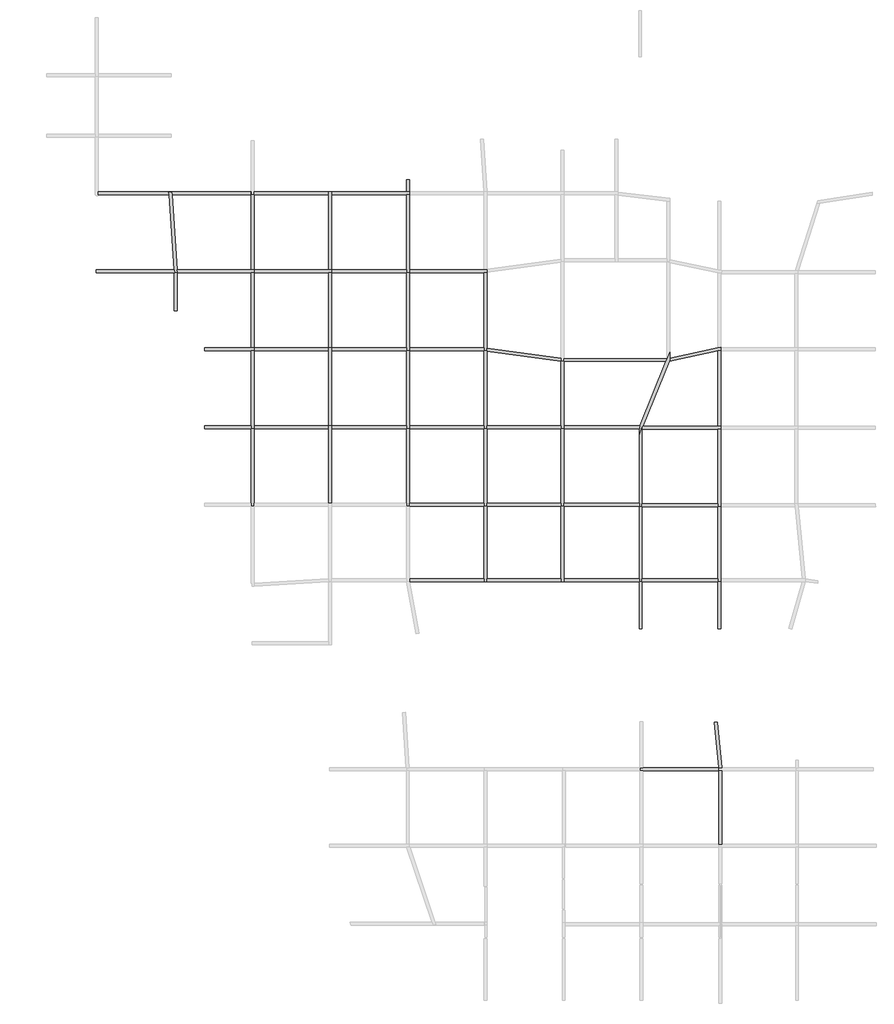
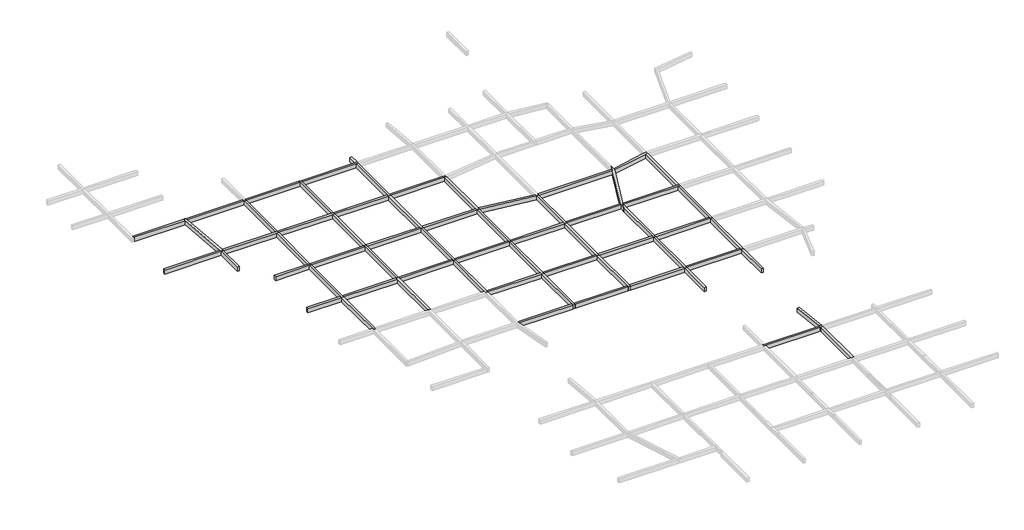
# One storey, part 2 of 8: 64 beams.
"""IFC4 building model written with IfcOpenShell, lengths in millimetres."""

from ifc_helpers import new_model, si_unit, frame, origin, place, context, project, spatial, polyline, outline, extrude, faceted_brep, element, save

model = new_model("IFC4")

# Units and contexts
model_context = context("Model", 3, world=origin())
ifc_project = project(units=[si_unit("LENGTHUNIT", "METRE", prefix="MILLI")], contexts=[model_context])

# Site, building, storey
site = spatial("IfcSite", under=ifc_project)
building = spatial("IfcBuilding", under=site)
storey = spatial("IfcBuildingStorey", under=building, Name="层高", Elevation=3300.0)

# Beams
placement = place(None, origin())
element("IfcBeam", 1, ObjectType="混凝土 - 矩形梁 : KL_beam", at=placement, inside=storey, context=model_context, shape_type="Brep", body=[
    faceted_brep([(70180.9452484, 119135.802002, 3300.0), (70480.2144635, 119156.7289441, 3300.0), (70460.6997743, 119435.802002, 3300.0), (69929.2560035, 127035.802002, 3300.0), (69908.2779599, 127335.802002, 3300.0), (69609.0087449, 127314.8750599, 3300.0), (69628.5234341, 127035.802002, 3300.0), (70159.9672049, 119435.802002, 3300.0), (70180.9452484, 119135.802002, 2700.0), (69609.0087449, 127314.8750599, 2700.0), (69628.5234341, 127035.802002, 2700.0), (70159.9672049, 119435.802002, 2700.0), (70480.2144635, 119156.7289441, 2700.0), (69908.2779599, 127335.802002, 2700.0), (69929.2560035, 127035.802002, 2700.0), (70460.6997743, 119435.802002, 2700.0)], [[[0, 1, 2, 3, 4, 5, 6, 7]], [[8, 0, 7, 6, 5, 9, 10, 11]], [[12, 8, 11, 10, 9, 13, 14, 15]], [[1, 12, 15, 14, 13, 4, 3, 2]], [[4, 13, 9, 5]], [[1, 0, 8, 12]]]),
])
element("IfcBeam", 2, ObjectType="混凝土 - 矩形梁 : KL_beam", at=placement, inside=storey, context=model_context, shape_type="Brep", body=[
    faceted_brep([(62233.8430954, 119135.802002, 3300.0), (70170.8225114, 119135.802002, 3300.0), (70180.9452484, 119135.802002, 3300.0), (70159.9672049, 119435.802002, 3300.0), (62233.8430954, 119435.802002, 3300.0), (62233.8430954, 119435.802002, 2700.0), (70159.9672049, 119435.802002, 2700.0), (70180.9452484, 119135.802002, 2700.0), (70170.8225114, 119135.802002, 2700.0), (62233.8430954, 119135.802002, 2700.0)], [[[0, 1, 2, 3, 4]], [[5, 4, 3, 6]], [[7, 8, 9, 5, 6]], [[2, 1, 0, 9, 8, 7]], [[0, 4, 5, 9]], [[3, 2, 7, 6]]]),
])
element("IfcBeam", 3, ObjectType="混凝土 - 矩形梁 : KL_beam", at=placement, inside=storey, context=model_context, shape_type="Brep", body=[
    faceted_brep([(70460.6997743, 119435.802002, 3300.0), (70480.2144635, 119156.7289441, 3300.0), (70180.9452484, 119135.802002, 3300.0), (70470.8225114, 119135.802002, 3300.0), (77970.8225114, 119135.802002, 3300.0), (78270.8225114, 119135.802002, 3300.0), (78270.8225114, 119435.802002, 3300.0), (77970.8225114, 119435.802002, 3300.0), (78270.8225114, 119135.802002, 2700.0), (70180.9452484, 119135.802002, 2700.0), (70470.8225114, 119135.802002, 2700.0), (77970.8225114, 119135.802002, 2700.0), (70480.2144635, 119156.7289441, 2700.0), (70460.6997743, 119435.802002, 2700.0), (77970.8225114, 119435.802002, 2700.0), (78270.8225114, 119435.802002, 2700.0)], [[[0, 1, 2, 3, 4, 5, 6, 7]], [[8, 5, 4, 3, 2, 9, 10, 11]], [[12, 13, 14, 15, 8, 11, 10, 9]], [[13, 0, 7, 6, 15, 14]], [[12, 1, 0, 13]], [[1, 12, 9, 2]], [[6, 5, 8, 15]]]),
])
element("IfcBeam", 4, ObjectType="混凝土 - 矩形梁 : KL_beam", at=placement, inside=storey, context=model_context, shape_type="Brep", body=[
    faceted_brep([(77970.8225114, 119435.802002, 3300.0), (78270.8225114, 119435.802002, 3300.0), (78270.8225114, 127035.802002, 3300.0), (77992.6046485, 127035.802002, 3300.0), (77992.6046485, 127335.802002, 3300.0), (77970.8225114, 127335.802002, 3300.0), (77970.8225114, 127035.802002, 3300.0), (78270.8225114, 119435.802002, 2700.0), (78270.8225114, 127035.802002, 2700.0), (77970.8225114, 119435.802002, 2700.0), (77970.8225114, 127035.802002, 2700.0), (77970.8225114, 127335.802002, 2700.0), (77992.6046485, 127335.802002, 2700.0), (77992.6046485, 127035.802002, 2700.0)], [[[0, 1, 2, 3, 4, 5, 6]], [[1, 7, 8, 2]], [[7, 9, 10, 11, 12, 13, 8]], [[5, 11, 10, 9, 0, 6]], [[3, 13, 12, 4]], [[1, 0, 9, 7]], [[11, 5, 4, 12]], [[13, 3, 2, 8]]]),
])
element("IfcBeam", 5, ObjectType="混凝土 - 矩形梁 : KL_beam", at=placement, inside=storey, context=model_context, shape_type="Brep", body=[
    faceted_brep([(86170.8225114, 119135.802002, 3300.0), (86170.8225114, 119435.802002, 3300.0), (85870.8225114, 119435.802002, 3300.0), (78270.8225114, 119435.802002, 3300.0), (78270.8225114, 119135.802002, 3300.0), (85870.8225114, 119135.802002, 3300.0), (86170.8225114, 119135.802002, 2700.0), (78270.8225114, 119135.802002, 2700.0), (85870.8225114, 119135.802002, 2700.0), (86170.8225114, 119435.802002, 2700.0), (78270.8225114, 119435.802002, 2700.0), (85870.8225114, 119435.802002, 2700.0)], [[[0, 1, 2, 3, 4, 5]], [[6, 0, 5, 4, 7, 8]], [[9, 6, 8, 7, 10, 11]], [[1, 9, 11, 10, 3, 2]], [[4, 3, 10, 7]], [[1, 0, 6, 9]]]),
])
element("IfcBeam", 6, ObjectType="混凝土 - 矩形梁 : KL_beam", at=placement, inside=storey, context=model_context, shape_type="Brep", body=[
    faceted_brep([(86170.8225114, 127335.802002, 3300.0), (85870.8225114, 127335.802002, 3300.0), (85870.8225114, 127035.802002, 3300.0), (85870.8225114, 119435.802002, 3300.0), (86170.8225114, 119435.802002, 3300.0), (86170.8225114, 127035.802002, 3300.0), (86170.8225114, 127335.802002, 2700.0), (86170.8225114, 119435.802002, 2700.0), (86170.8225114, 127035.802002, 2700.0), (85870.8225114, 127335.802002, 2700.0), (85870.8225114, 119435.802002, 2700.0), (85870.8225114, 127035.802002, 2700.0)], [[[0, 1, 2, 3, 4, 5]], [[6, 0, 5, 4, 7, 8]], [[9, 6, 8, 7, 10, 11]], [[1, 9, 11, 10, 3, 2]], [[4, 3, 10, 7]], [[1, 0, 6, 9]]]),
])
element("IfcBeam", 7, ObjectType="混凝土 - 矩形梁 : KL_beam", at=placement, inside=storey, context=model_context, shape_type="Brep", body=[
    faceted_brep([(94070.8225114, 127035.802002, 3300.0), (94070.8225114, 127335.802002, 3300.0), (93770.8225114, 127335.802002, 3300.0), (86170.8225114, 127335.802002, 3300.0), (86170.8225114, 127035.802002, 3300.0), (93770.8225114, 127035.802002, 3300.0), (94070.8225114, 127035.802002, 2700.0), (86170.8225114, 127035.802002, 2700.0), (93770.8225114, 127035.802002, 2700.0), (94070.8225114, 127335.802002, 2700.0), (86170.8225114, 127335.802002, 2700.0), (93770.8225114, 127335.802002, 2700.0)], [[[0, 1, 2, 3, 4, 5]], [[6, 0, 5, 4, 7, 8]], [[9, 6, 8, 7, 10, 11]], [[1, 9, 11, 10, 3, 2]], [[4, 3, 10, 7]], [[1, 0, 6, 9]]]),
])
element("IfcBeam", 8, ObjectType="混凝土 - 矩形梁 : KL_beam", at=placement, inside=storey, context=model_context, shape_type="Brep", body=[
    faceted_brep([(93770.8225114, 119135.802002, 3300.0), (94070.8225114, 119135.802002, 3300.0), (94070.8225114, 119435.802002, 3300.0), (94070.8225114, 127035.802002, 3300.0), (93770.8225114, 127035.802002, 3300.0), (93770.8225114, 119435.802002, 3300.0), (93770.8225114, 119135.802002, 2700.0), (93770.8225114, 127035.802002, 2700.0), (93770.8225114, 119435.802002, 2700.0), (94070.8225114, 119135.802002, 2700.0), (94070.8225114, 127035.802002, 2700.0), (94070.8225114, 119435.802002, 2700.0)], [[[0, 1, 2, 3, 4, 5]], [[6, 0, 5, 4, 7, 8]], [[9, 6, 8, 7, 10, 11]], [[1, 9, 11, 10, 3, 2]], [[4, 3, 10, 7]], [[1, 0, 6, 9]]]),
])
element("IfcBeam", 9, ObjectType="混凝土 - 矩形梁 : KL_beam", at=placement, inside=storey, context=model_context, shape_type="SweptSolid", body=[
    extrude(outline(polyline([(86170.8225114, 119135.802002), (86170.8225114, 119435.802002), (93770.8225114, 119435.802002), (93770.8225114, 119135.802002), (86170.8225114, 119135.802002)])), frame((0.0, 0.0, 2700.0), z_axis=(0.0, 0.0, 1.0), x_axis=(1.0, 0.0, 0.0)), (0.0, 0.0, 1.0), 600.0),
])
element("IfcBeam", 10, ObjectType="混凝土 - 矩形梁 : KL_beam", at=placement, inside=storey, context=model_context, shape_type="Brep", body=[
    faceted_brep([(101970.8225114, 119135.802002, 3300.0), (101970.8225114, 119155.4715744, 3300.0), (101970.8225114, 119435.802002, 3300.0), (101670.8225114, 119435.802002, 3300.0), (94070.8225114, 119435.802002, 3300.0), (94070.8225114, 119135.802002, 3300.0), (101670.8225114, 119135.802002, 3300.0), (101970.8225114, 119135.802002, 2700.0), (94070.8225114, 119135.802002, 2700.0), (101670.8225114, 119135.802002, 2700.0), (101970.8225114, 119435.802002, 2700.0), (101970.8225114, 119155.4715744, 2700.0), (94070.8225114, 119435.802002, 2700.0), (101670.8225114, 119435.802002, 2700.0)], [[[0, 1, 2, 3, 4, 5, 6]], [[7, 0, 6, 5, 8, 9]], [[10, 11, 7, 9, 8, 12, 13]], [[2, 10, 13, 12, 4, 3]], [[5, 4, 12, 8]], [[2, 1, 0, 7, 11, 10]]]),
])
element("IfcBeam", 11, ObjectType="混凝土 - 矩形梁 : KL_beam", at=placement, inside=storey, context=model_context, shape_type="SweptSolid", body=[
    extrude(outline(polyline([(93770.8225114, 128593.2738083), (94070.8225114, 128593.2738083), (94070.8225114, 127335.802002), (93770.8225114, 127335.802002), (93770.8225114, 128593.2738083)])), frame((0.0, 0.0, 2700.0), z_axis=(0.0, 0.0, 1.0), x_axis=(1.0, 0.0, 0.0)), (0.0, 0.0, 1.0), 600.0),
])
element("IfcBeam", 12, ObjectType="混凝土 - 矩形梁 : KL_beam", at=placement, inside=storey, context=model_context, shape_type="Brep", body=[
    faceted_brep([(70170.8225114, 115247.0451941, 3300.0), (70470.8225114, 115247.0451941, 3300.0), (70470.8225114, 119135.802002, 3300.0), (70180.9452484, 119135.802002, 3300.0), (70170.8225114, 119135.802002, 3300.0), (70170.8225114, 115247.0451941, 2700.0), (70170.8225114, 119135.802002, 2700.0), (70470.8225114, 115247.0451941, 2700.0), (70180.9452484, 119135.802002, 2700.0), (70470.8225114, 119135.802002, 2700.0)], [[[0, 1, 2, 3, 4]], [[5, 0, 4, 6]], [[7, 5, 6, 8, 9]], [[1, 7, 9, 2]], [[1, 0, 5, 7]], [[2, 9, 8, 6, 4, 3]]]),
])
element("IfcBeam", 13, ObjectType="混凝土 - 矩形梁 : KL_beam", at=placement, inside=storey, context=model_context, shape_type="Brep", body=[
    faceted_brep([(78270.8225114, 111177.0451941, 3300.0), (78270.8225114, 111477.0451941, 3300.0), (77970.8225114, 111477.0451941, 3300.0), (73233.8430954, 111477.0451941, 3300.0), (73233.8430954, 111177.0451941, 3300.0), (77970.8225114, 111177.0451941, 3300.0), (78270.8225114, 111177.0451941, 2700.0), (73233.8430954, 111177.0451941, 2700.0), (77970.8225114, 111177.0451941, 2700.0), (78270.8225114, 111477.0451941, 2700.0), (73233.8430954, 111477.0451941, 2700.0), (77970.8225114, 111477.0451941, 2700.0)], [[[0, 1, 2, 3, 4, 5]], [[6, 0, 5, 4, 7, 8]], [[9, 6, 8, 7, 10, 11]], [[1, 9, 11, 10, 3, 2]], [[4, 3, 10, 7]], [[1, 0, 6, 9]]]),
])
element("IfcBeam", 14, ObjectType="混凝土 - 矩形梁 : KL_beam", at=placement, inside=storey, context=model_context, shape_type="SweptSolid", body=[
    extrude(outline(polyline([(77970.8225114, 119135.802002), (78270.8225114, 119135.802002), (78270.8225114, 111477.0451941), (77970.8225114, 111477.0451941), (77970.8225114, 119135.802002)])), frame((0.0, 0.0, 2700.0), z_axis=(0.0, 0.0, 1.0), x_axis=(1.0, 0.0, 0.0)), (0.0, 0.0, 1.0), 600.0),
])
element("IfcBeam", 15, ObjectType="混凝土 - 矩形梁 : KL_beam", at=placement, inside=storey, context=model_context, shape_type="Brep", body=[
    faceted_brep([(77970.8225114, 103277.0451941, 3300.0), (78270.8225114, 103277.0451941, 3300.0), (78270.8225114, 103577.0451941, 3300.0), (78270.8225114, 111177.0451941, 3300.0), (77970.8225114, 111177.0451941, 3300.0), (77970.8225114, 103577.0451941, 3300.0), (77970.8225114, 103277.0451941, 2700.0), (77970.8225114, 111177.0451941, 2700.0), (77970.8225114, 103577.0451941, 2700.0), (78270.8225114, 103277.0451941, 2700.0), (78270.8225114, 111177.0451941, 2700.0), (78270.8225114, 103577.0451941, 2700.0)], [[[0, 1, 2, 3, 4, 5]], [[6, 0, 5, 4, 7, 8]], [[9, 6, 8, 7, 10, 11]], [[1, 9, 11, 10, 3, 2]], [[4, 3, 10, 7]], [[1, 0, 6, 9]]]),
])
element("IfcBeam", 16, ObjectType="混凝土 - 矩形梁 : KL_beam", at=placement, inside=storey, context=model_context, shape_type="SweptSolid", body=[
    extrude(outline(polyline([(73233.8430954, 103277.0451941), (73233.8430954, 103577.0451941), (77970.8225114, 103577.0451941), (77970.8225114, 103277.0451941), (73233.8430954, 103277.0451941)])), frame((0.0, 0.0, 2700.0), z_axis=(0.0, 0.0, 1.0), x_axis=(1.0, 0.0, 0.0)), (0.0, 0.0, 1.0), 600.0),
])
element("IfcBeam", 17, ObjectType="混凝土 - 矩形梁 : KL_beam", at=placement, inside=storey, context=model_context, shape_type="Brep", body=[
    faceted_brep([(77970.8225114, 95377.0451941, 3300.0), (78270.8225114, 95377.0451941, 3300.0), (78270.8225114, 95677.0451941, 3300.0), (78270.8225114, 103277.0451941, 3300.0), (77970.8225114, 103277.0451941, 3300.0), (77970.8225114, 95677.0451941, 3300.0), (77970.8225114, 95377.0451941, 2700.0), (77970.8225114, 103277.0451941, 2700.0), (77970.8225114, 95677.0451941, 2700.0), (78270.8225114, 95377.0451941, 2700.0), (78270.8225114, 103277.0451941, 2700.0), (78270.8225114, 95677.0451941, 2700.0)], [[[0, 1, 2, 3, 4, 5]], [[6, 0, 5, 4, 7, 8]], [[9, 6, 8, 7, 10, 11]], [[1, 9, 11, 10, 3, 2]], [[4, 3, 10, 7]], [[1, 0, 6, 9]]]),
])
element("IfcBeam", 18, ObjectType="混凝土 - 矩形梁 : KL_beam", at=placement, inside=storey, context=model_context, shape_type="Brep", body=[
    faceted_brep([(86170.8225114, 103577.0451941, 3300.0), (85870.8225114, 103577.0451941, 3300.0), (85870.8225114, 103277.0451941, 3300.0), (85870.8225114, 95677.0451941, 3300.0), (86170.8225114, 95677.0451941, 3300.0), (86170.8225114, 103277.0451941, 3300.0), (86170.8225114, 103577.0451941, 2700.0), (86170.8225114, 95677.0451941, 2700.0), (86170.8225114, 103277.0451941, 2700.0), (85870.8225114, 103577.0451941, 2700.0), (85870.8225114, 95677.0451941, 2700.0), (85870.8225114, 103277.0451941, 2700.0)], [[[0, 1, 2, 3, 4, 5]], [[6, 0, 5, 4, 7, 8]], [[9, 6, 8, 7, 10, 11]], [[1, 9, 11, 10, 3, 2]], [[1, 0, 6, 9]], [[4, 3, 10, 7]]]),
])
element("IfcBeam", 19, ObjectType="混凝土 - 矩形梁 : KL_beam", at=placement, inside=storey, context=model_context, shape_type="Brep", body=[
    faceted_brep([(86170.8225114, 111477.0451941, 3300.0), (85870.8225114, 111477.0451941, 3300.0), (85870.8225114, 111177.0451941, 3300.0), (85870.8225114, 103577.0451941, 3300.0), (86170.8225114, 103577.0451941, 3300.0), (86170.8225114, 111177.0451941, 3300.0), (86170.8225114, 111477.0451941, 2700.0), (86170.8225114, 103577.0451941, 2700.0), (86170.8225114, 111177.0451941, 2700.0), (85870.8225114, 111477.0451941, 2700.0), (85870.8225114, 103577.0451941, 2700.0), (85870.8225114, 111177.0451941, 2700.0)], [[[0, 1, 2, 3, 4, 5]], [[6, 0, 5, 4, 7, 8]], [[9, 6, 8, 7, 10, 11]], [[1, 9, 11, 10, 3, 2]], [[1, 0, 6, 9]], [[4, 3, 10, 7]]]),
])
element("IfcBeam", 20, ObjectType="混凝土 - 矩形梁 : KL_beam", at=placement, inside=storey, context=model_context, shape_type="SweptSolid", body=[
    extrude(outline(polyline([(85870.8225114, 119135.802002), (86170.8225114, 119135.802002), (86170.8225114, 111477.0451941), (85870.8225114, 111477.0451941), (85870.8225114, 119135.802002)])), frame((0.0, 0.0, 2700.0), z_axis=(0.0, 0.0, 1.0), x_axis=(1.0, 0.0, 0.0)), (0.0, 0.0, 1.0), 600.0),
])
element("IfcBeam", 21, ObjectType="混凝土 - 矩形梁 : KL_beam", at=placement, inside=storey, context=model_context, shape_type="Brep", body=[
    faceted_brep([(93770.8225114, 111177.0451941, 3300.0), (94070.8225114, 111177.0451941, 3300.0), (94070.8225114, 111477.0451941, 3300.0), (94070.8225114, 119135.802002, 3300.0), (93770.8225114, 119135.802002, 3300.0), (93770.8225114, 111477.0451941, 3300.0), (93770.8225114, 111177.0451941, 2700.0), (93770.8225114, 119135.802002, 2700.0), (93770.8225114, 111477.0451941, 2700.0), (94070.8225114, 111177.0451941, 2700.0), (94070.8225114, 119135.802002, 2700.0), (94070.8225114, 111477.0451941, 2700.0)], [[[0, 1, 2, 3, 4, 5]], [[6, 0, 5, 4, 7, 8]], [[9, 6, 8, 7, 10, 11]], [[1, 9, 11, 10, 3, 2]], [[4, 3, 10, 7]], [[1, 0, 6, 9]]]),
])
element("IfcBeam", 22, ObjectType="混凝土 - 矩形梁 : KL_beam", at=placement, inside=storey, context=model_context, shape_type="Brep", body=[
    faceted_brep([(93770.8225114, 103277.0451941, 3300.0), (94070.8225114, 103277.0451941, 3300.0), (94070.8225114, 103577.0451941, 3300.0), (94070.8225114, 111177.0451941, 3300.0), (93770.8225114, 111177.0451941, 3300.0), (93770.8225114, 103577.0451941, 3300.0), (93770.8225114, 103277.0451941, 2700.0), (93770.8225114, 111177.0451941, 2700.0), (93770.8225114, 103577.0451941, 2700.0), (94070.8225114, 103277.0451941, 2700.0), (94070.8225114, 111177.0451941, 2700.0), (94070.8225114, 103577.0451941, 2700.0)], [[[0, 1, 2, 3, 4, 5]], [[6, 0, 5, 4, 7, 8]], [[9, 6, 8, 7, 10, 11]], [[1, 9, 11, 10, 3, 2]], [[4, 3, 10, 7]], [[1, 0, 6, 9]]]),
])
element("IfcBeam", 23, ObjectType="混凝土 - 矩形梁 : KL_beam", at=placement, inside=storey, context=model_context, shape_type="Brep", body=[
    faceted_brep([(93770.8225114, 95377.0451941, 3300.0), (94070.8225114, 95377.0451941, 3300.0), (94070.8225114, 95677.0451941, 3300.0), (94070.8225114, 103277.0451941, 3300.0), (93770.8225114, 103277.0451941, 3300.0), (93770.8225114, 95677.0451941, 3300.0), (93770.8225114, 95377.0451941, 2700.0), (93770.8225114, 103277.0451941, 2700.0), (93770.8225114, 95677.0451941, 2700.0), (94070.8225114, 95377.0451941, 2700.0), (94070.8225114, 103277.0451941, 2700.0), (94070.8225114, 95677.0451941, 2700.0)], [[[0, 1, 2, 3, 4, 5]], [[6, 0, 5, 4, 7, 8]], [[9, 6, 8, 7, 10, 11]], [[1, 9, 11, 10, 3, 2]], [[4, 3, 10, 7]], [[1, 0, 6, 9]]]),
])
element("IfcBeam", 24, ObjectType="混凝土 - 矩形梁 : KL_beam", at=placement, inside=storey, context=model_context, shape_type="Brep", body=[
    faceted_brep([(101670.8225114, 111177.0451941, 3300.0), (101970.8225114, 111177.0451941, 3300.0), (101970.8225114, 111457.869772, 3300.0), (101970.8225114, 119135.802002, 3300.0), (101670.8225114, 119135.802002, 3300.0), (101670.8225114, 111477.0451941, 3300.0), (101670.8225114, 111177.0451941, 2700.0), (101670.8225114, 119135.802002, 2700.0), (101670.8225114, 111477.0451941, 2700.0), (101970.8225114, 111177.0451941, 2700.0), (101970.8225114, 119135.802002, 2700.0), (101970.8225114, 111457.869772, 2700.0)], [[[0, 1, 2, 3, 4, 5]], [[6, 0, 5, 4, 7, 8]], [[9, 6, 8, 7, 10, 11]], [[1, 9, 11, 10, 3, 2]], [[4, 3, 10, 7]], [[1, 0, 6, 9]]]),
])
element("IfcBeam", 25, ObjectType="混凝土 - 矩形梁 : KL_beam", at=placement, inside=storey, context=model_context, shape_type="Brep", body=[
    faceted_brep([(101670.8225114, 103277.0451941, 3300.0), (101970.8225114, 103277.0451941, 3300.0), (101970.8225114, 103577.0451941, 3300.0), (101970.8225114, 111155.0591624, 3300.0), (101970.8225114, 111177.0451941, 3300.0), (101670.8225114, 111177.0451941, 3300.0), (101670.8225114, 103577.0451941, 3300.0), (101670.8225114, 103277.0451941, 2700.0), (101670.8225114, 111177.0451941, 2700.0), (101670.8225114, 103577.0451941, 2700.0), (101970.8225114, 103277.0451941, 2700.0), (101970.8225114, 111177.0451941, 2700.0), (101970.8225114, 111155.0591624, 2700.0), (101970.8225114, 103577.0451941, 2700.0)], [[[0, 1, 2, 3, 4, 5, 6]], [[7, 0, 6, 5, 8, 9]], [[10, 7, 9, 8, 11, 12, 13]], [[1, 10, 13, 12, 11, 4, 3, 2]], [[5, 4, 11, 8]], [[1, 0, 7, 10]]]),
])
element("IfcBeam", 26, ObjectType="混凝土 - 矩形梁 : KL_beam", at=placement, inside=storey, context=model_context, shape_type="Brep", body=[
    faceted_brep([(101670.8225114, 95377.0451941, 3300.0), (101970.8225114, 95377.0451941, 3300.0), (101970.8225114, 95677.0451941, 3300.0), (101970.8225114, 103277.0451941, 3300.0), (101670.8225114, 103277.0451941, 3300.0), (101670.8225114, 95677.0451941, 3300.0), (101670.8225114, 95377.0451941, 2700.0), (101670.8225114, 103277.0451941, 2700.0), (101670.8225114, 95677.0451941, 2700.0), (101970.8225114, 95377.0451941, 2700.0), (101970.8225114, 103277.0451941, 2700.0), (101970.8225114, 95677.0451941, 2700.0)], [[[0, 1, 2, 3, 4, 5]], [[6, 0, 5, 4, 7, 8]], [[9, 6, 8, 7, 10, 11]], [[1, 9, 11, 10, 3, 2]], [[4, 3, 10, 7]], [[1, 0, 6, 9]]]),
])
element("IfcBeam", 27, ObjectType="混凝土 - 矩形梁 : KL_beam", at=placement, inside=storey, context=model_context, shape_type="Brep", body=[
    faceted_brep([(101670.8225114, 87731.7102801, 3300.0), (101970.8225114, 87731.7102801, 3300.0), (101970.8225114, 88031.7102801, 3300.0), (101970.8225114, 95377.0451941, 3300.0), (101670.8225114, 95377.0451941, 3300.0), (101670.8225114, 88031.7102801, 3300.0), (101670.8225114, 87731.7102801, 2700.0), (101670.8225114, 95377.0451941, 2700.0), (101670.8225114, 88031.7102801, 2700.0), (101970.8225114, 87731.7102801, 2700.0), (101970.8225114, 95377.0451941, 2700.0), (101970.8225114, 88031.7102801, 2700.0)], [[[0, 1, 2, 3, 4, 5]], [[6, 0, 5, 4, 7, 8]], [[9, 6, 8, 7, 10, 11]], [[1, 9, 11, 10, 3, 2]], [[4, 3, 10, 7]], [[1, 0, 6, 9]]]),
])
element("IfcBeam", 28, ObjectType="混凝土 - 矩形梁 : KL_beam", at=placement, inside=storey, context=model_context, shape_type="Brep", body=[
    faceted_brep([(109470.8225114, 103277.0451941, 3300.0), (109770.8225114, 103277.0451941, 3300.0), (109770.8225114, 103577.0451941, 3300.0), (109770.8225114, 110106.8473936, 3300.0), (109470.8225114, 110106.8473936, 3300.0), (109470.8225114, 103577.0451941, 3300.0), (109470.8225114, 103277.0451941, 2700.0), (109470.8225114, 110106.8473936, 2700.0), (109470.8225114, 103577.0451941, 2700.0), (109770.8225114, 103277.0451941, 2700.0), (109770.8225114, 110106.8473936, 2700.0), (109770.8225114, 103577.0451941, 2700.0)], [[[0, 1, 2, 3, 4, 5]], [[6, 0, 5, 4, 7, 8]], [[9, 6, 8, 7, 10, 11]], [[1, 9, 11, 10, 3, 2]], [[4, 3, 10, 7]], [[1, 0, 6, 9]]]),
])
element("IfcBeam", 29, ObjectType="混凝土 - 矩形梁 : KL_beam", at=placement, inside=storey, context=model_context, shape_type="Brep", body=[
    faceted_brep([(109470.8225114, 95377.0451941, 3300.0), (109770.8225114, 95377.0451941, 3300.0), (109770.8225114, 95677.0451941, 3300.0), (109770.8225114, 103277.0451941, 3300.0), (109470.8225114, 103277.0451941, 3300.0), (109470.8225114, 95677.0451941, 3300.0), (109470.8225114, 95377.0451941, 2700.0), (109470.8225114, 103277.0451941, 2700.0), (109470.8225114, 95677.0451941, 2700.0), (109770.8225114, 95377.0451941, 2700.0), (109770.8225114, 103277.0451941, 2700.0), (109770.8225114, 95677.0451941, 2700.0)], [[[0, 1, 2, 3, 4, 5]], [[6, 0, 5, 4, 7, 8]], [[9, 6, 8, 7, 10, 11]], [[1, 9, 11, 10, 3, 2]], [[4, 3, 10, 7]], [[1, 0, 6, 9]]]),
])
element("IfcBeam", 30, ObjectType="混凝土 - 矩形梁 : KL_beam", at=placement, inside=storey, context=model_context, shape_type="Brep", body=[
    faceted_brep([(109470.8225114, 87731.7102801, 3300.0), (109770.8225114, 87731.7102801, 3300.0), (109770.8225114, 88031.7102801, 3300.0), (109770.8225114, 95377.0451941, 3300.0), (109470.8225114, 95377.0451941, 3300.0), (109470.8225114, 88031.7102801, 3300.0), (109470.8225114, 87731.7102801, 2700.0), (109470.8225114, 95377.0451941, 2700.0), (109470.8225114, 88031.7102801, 2700.0), (109770.8225114, 87731.7102801, 2700.0), (109770.8225114, 95377.0451941, 2700.0), (109770.8225114, 88031.7102801, 2700.0)], [[[0, 1, 2, 3, 4, 5]], [[6, 0, 5, 4, 7, 8]], [[9, 6, 8, 7, 10, 11]], [[1, 9, 11, 10, 3, 2]], [[4, 3, 10, 7]], [[1, 0, 6, 9]]]),
])
element("IfcBeam", 31, ObjectType="混凝土 - 矩形梁 : KL_beam", at=placement, inside=storey, context=model_context, shape_type="Brep", body=[
    faceted_brep([(117426.2900999, 103411.1618028, 3300.0), (117426.2900999, 103277.0451941, 3300.0), (117426.2900999, 102617.7429892, 3300.0), (117726.2900999, 103352.2587574, 3300.0), (117799.5839067, 103531.7102801, 3300.0), (120493.1632599, 110126.6319733, 3300.0), (120534.3184952, 110227.3958709, 3300.0), (120534.3184952, 110442.081967, 3300.0), (120534.3184952, 111020.8146845, 3300.0), (120234.3184952, 110286.2989162, 3300.0), (120161.0246884, 110106.8473936, 3300.0), (117494.0422429, 103577.0451941, 3300.0), (117426.2900999, 103411.1618028, 2700.0), (120534.3184952, 111020.8146845, 2700.0), (120234.3184952, 110286.2989162, 2700.0), (120161.0246884, 110106.8473936, 2700.0), (117494.0422429, 103577.0451941, 2700.0), (117426.2900999, 102617.7429892, 2700.0), (117426.2900999, 103277.0451941, 2700.0), (120534.3184952, 110442.081967, 2700.0), (120534.3184952, 110227.3958709, 2700.0), (120493.1632599, 110126.6319733, 2700.0), (117799.5839067, 103531.7102801, 2700.0), (117726.2900999, 103352.2587574, 2700.0)], [[[0, 1, 2, 3, 4, 5, 6, 7, 8, 9, 10, 11]], [[12, 0, 11, 10, 9, 8, 13, 14, 15, 16]], [[17, 18, 12, 16, 15, 14, 13, 19, 20, 21, 22, 23]], [[2, 17, 23, 22, 21, 20, 6, 5, 4, 3]], [[2, 1, 0, 12, 18, 17]], [[8, 7, 6, 20, 19, 13]]]),
])
element("IfcBeam", 32, ObjectType="混凝土 - 矩形梁 : KL_beam", at=placement, inside=storey, context=model_context, shape_type="Brep", body=[
    faceted_brep([(117426.2900999, 95331.7102801, 3300.0), (117726.2900999, 95331.7102801, 3300.0), (117726.2900999, 95631.7102801, 3300.0), (117726.2900999, 103231.7102801, 3300.0), (117726.2900999, 103352.2587574, 3300.0), (117426.2900999, 102617.7429892, 3300.0), (117426.2900999, 95677.0451941, 3300.0), (117426.2900999, 95377.0451941, 3300.0), (117426.2900999, 95331.7102801, 2700.0), (117426.2900999, 102617.7429892, 2700.0), (117426.2900999, 95677.0451941, 2700.0), (117426.2900999, 95377.0451941, 2700.0), (117726.2900999, 95331.7102801, 2700.0), (117726.2900999, 103352.2587574, 2700.0), (117726.2900999, 103231.7102801, 2700.0), (117726.2900999, 95631.7102801, 2700.0)], [[[0, 1, 2, 3, 4, 5, 6, 7]], [[8, 0, 7, 6, 5, 9, 10, 11]], [[12, 8, 11, 10, 9, 13, 14, 15]], [[1, 12, 15, 14, 13, 4, 3, 2]], [[5, 4, 13, 9]], [[1, 0, 8, 12]]]),
])
element("IfcBeam", 33, ObjectType="混凝土 - 矩形梁 : KL_beam", at=placement, inside=storey, context=model_context, shape_type="Brep", body=[
    faceted_brep([(117426.2900999, 87731.7102801, 3300.0), (117726.2900999, 87731.7102801, 3300.0), (117726.2900999, 88031.7102801, 3300.0), (117726.2900999, 95331.7102801, 3300.0), (117426.2900999, 95331.7102801, 3300.0), (117426.2900999, 88031.7102801, 3300.0), (117426.2900999, 87731.7102801, 2700.0), (117426.2900999, 95331.7102801, 2700.0), (117426.2900999, 88031.7102801, 2700.0), (117726.2900999, 87731.7102801, 2700.0), (117726.2900999, 95331.7102801, 2700.0), (117726.2900999, 88031.7102801, 2700.0)], [[[0, 1, 2, 3, 4, 5]], [[6, 0, 5, 4, 7, 8]], [[9, 6, 8, 7, 10, 11]], [[1, 9, 11, 10, 3, 2]], [[4, 3, 10, 7]], [[1, 0, 6, 9]]]),
])
element("IfcBeam", 34, ObjectType="混凝土 - 矩形梁 : KL_beam", at=placement, inside=storey, context=model_context, shape_type="SweptSolid", body=[
    extrude(outline(polyline([(117726.2900999, 82948.5269181), (117426.2900999, 82948.5269181), (117426.2900999, 87731.7102801), (117726.2900999, 87731.7102801), (117726.2900999, 82948.5269181)])), frame((0.0, 0.0, 2700.0), z_axis=(0.0, 0.0, 1.0), x_axis=(1.0, 0.0, 0.0)), (0.0, 0.0, 1.0), 600.0),
])
element("IfcBeam", 35, ObjectType="混凝土 - 矩形梁 : KL_beam", at=placement, inside=storey, context=model_context, shape_type="SweptSolid", body=[
    extrude(outline(polyline([(109770.8225114, 110106.8473936), (109770.8225114, 110406.8473936), (120234.3184952, 110406.8473936), (120234.3184952, 110286.2989162), (120161.0246884, 110106.8473936), (109770.8225114, 110106.8473936)])), frame((0.0, 0.0, 2700.0), z_axis=(0.0, 0.0, 1.0), x_axis=(1.0, 0.0, 0.0)), (0.0, 0.0, 1.0), 600.0),
])
element("IfcBeam", 36, ObjectType="混凝土 - 矩形梁 : KL_beam", at=placement, inside=storey, context=model_context, shape_type="Brep", body=[
    faceted_brep([(120534.3184952, 110227.3958709, 3300.0), (120493.1632599, 110126.6319733, 3300.0), (125448.8238726, 111179.9901539, 3300.0), (125748.8238726, 111243.7571224, 3300.0), (125748.8238726, 111515.2247274, 3300.0), (125748.8238726, 111550.4593009, 3300.0), (125448.8238726, 111486.6923324, 3300.0), (120534.3184952, 110442.081967, 3300.0), (120534.3184952, 110406.8473936, 3300.0), (120493.1632599, 110126.6319733, 2700.0), (125448.8238726, 111179.9901539, 2700.0), (125748.8238726, 111243.7571224, 2700.0), (120534.3184952, 110227.3958709, 2700.0), (120534.3184952, 110406.8473936, 2700.0), (120534.3184952, 110442.081967, 2700.0), (125448.8238726, 111486.6923324, 2700.0), (125748.8238726, 111550.4593009, 2700.0), (125748.8238726, 111515.2247274, 2700.0)], [[[0, 1, 2, 3, 4, 5, 6, 7, 8]], [[1, 9, 10, 11, 3, 2]], [[9, 12, 13, 14, 15, 16, 17, 11, 10]], [[14, 7, 6, 5, 16, 15]], [[0, 12, 9, 1]], [[12, 0, 8, 7, 14, 13]], [[5, 4, 3, 11, 17, 16]]]),
])
element("IfcBeam", 37, ObjectType="混凝土 - 矩形梁 : KL_beam", at=placement, inside=storey, context=model_context, shape_type="Brep", body=[
    faceted_brep([(125748.8238726, 103231.7102801, 3300.0), (125748.8238726, 103531.7102801, 3300.0), (125448.8238726, 103531.7102801, 3300.0), (117799.5839067, 103531.7102801, 3300.0), (117726.2900999, 103352.2587574, 3300.0), (117726.2900999, 103231.7102801, 3300.0), (125448.8238728, 103231.7102801, 3300.0), (125748.8238726, 103231.7102801, 2700.0), (117726.2900999, 103231.7102801, 2700.0), (125448.8238728, 103231.7102801, 2700.0), (125748.8238726, 103531.7102801, 2700.0), (117726.2900999, 103352.2587574, 2700.0), (117799.5839067, 103531.7102801, 2700.0), (125448.8238726, 103531.7102801, 2700.0)], [[[0, 1, 2, 3, 4, 5, 6]], [[7, 0, 6, 5, 8, 9]], [[10, 7, 9, 8, 11, 12, 13]], [[12, 3, 2, 1, 10, 13]], [[3, 12, 11, 4]], [[5, 4, 11, 8]], [[1, 0, 7, 10]]]),
])
element("IfcBeam", 38, ObjectType="混凝土 - 矩形梁 : KL_beam", at=placement, inside=storey, context=model_context, shape_type="Brep", body=[
    faceted_brep([(125748.8238726, 111243.7571224, 3300.0), (125448.8238726, 111179.9901539, 3300.0), (125448.8238726, 103531.7102801, 3300.0), (125748.8238726, 103531.7102801, 3300.0), (125748.8238726, 111215.2247274, 3300.0), (125448.8238726, 111179.9901539, 2700.0), (125448.8238726, 103531.7102801, 2700.0), (125748.8238726, 111243.7571224, 2700.0), (125748.8238726, 111215.2247274, 2700.0), (125748.8238726, 103531.7102801, 2700.0)], [[[0, 1, 2, 3, 4]], [[1, 5, 6, 2]], [[5, 7, 8, 9, 6]], [[7, 0, 4, 3, 9, 8]], [[1, 0, 7, 5]], [[3, 2, 6, 9]]]),
])
element("IfcBeam", 39, ObjectType="混凝土 - 矩形梁 : KL_beam", at=placement, inside=storey, context=model_context, shape_type="Brep", body=[
    faceted_brep([(125448.8238728, 95331.7102801, 3300.0), (125748.8238728, 95331.7102801, 3300.0), (125748.8238728, 95631.7102801, 3300.0), (125748.8238728, 103231.7102801, 3300.0), (125448.8238728, 103231.7102801, 3300.0), (125448.8238728, 95631.7102801, 3300.0), (125448.8238728, 95331.7102801, 2700.0), (125448.8238728, 103231.7102801, 2700.0), (125448.8238728, 95631.7102801, 2700.0), (125748.8238728, 95331.7102801, 2700.0), (125748.8238728, 103231.7102801, 2700.0), (125748.8238728, 95631.7102801, 2700.0)], [[[0, 1, 2, 3, 4, 5]], [[6, 0, 5, 4, 7, 8]], [[9, 6, 8, 7, 10, 11]], [[1, 9, 11, 10, 3, 2]], [[4, 3, 10, 7]], [[1, 0, 6, 9]]]),
])
element("IfcBeam", 40, ObjectType="混凝土 - 矩形梁 : KL_beam", at=placement, inside=storey, context=model_context, shape_type="SweptSolid", body=[
    extrude(outline(polyline([(117726.2900999, 95331.7102801), (117726.2900999, 95631.7102801), (125448.8238728, 95631.7102801), (125448.8238728, 95331.7102801), (117726.2900999, 95331.7102801)])), frame((0.0, 0.0, 2700.0), z_axis=(0.0, 0.0, 1.0), x_axis=(1.0, 0.0, 0.0)), (0.0, 0.0, 1.0), 600.0),
])
element("IfcBeam", 41, ObjectType="混凝土 - 矩形梁 : KL_beam", at=placement, inside=storey, context=model_context, shape_type="Brep", body=[
    faceted_brep([(125448.8238729, 87731.7102801, 3300.0), (125748.8238729, 87731.7102801, 3300.0), (125748.8238729, 88031.7102801, 3300.0), (125748.8238728, 95331.7102801, 3300.0), (125448.8238728, 95331.7102801, 3300.0), (125448.8238729, 88031.7102801, 3300.0), (125448.8238729, 87731.7102801, 2700.0), (125448.8238728, 95331.7102801, 2700.0), (125448.8238729, 88031.7102801, 2700.0), (125748.8238729, 87731.7102801, 2700.0), (125748.8238728, 95331.7102801, 2700.0), (125748.8238729, 88031.7102801, 2700.0)], [[[0, 1, 2, 3, 4, 5]], [[6, 0, 5, 4, 7, 8]], [[9, 6, 8, 7, 10, 11]], [[1, 9, 11, 10, 3, 2]], [[4, 3, 10, 7]], [[1, 0, 6, 9]]]),
])
element("IfcBeam", 42, ObjectType="混凝土 - 矩形梁 : KL_beam", at=placement, inside=storey, context=model_context, shape_type="SweptSolid", body=[
    extrude(outline(polyline([(117726.2900999, 87731.7102801), (117726.2900999, 88031.7102801), (125448.8238729, 88031.7102801), (125448.8238729, 87731.7102801), (117726.2900999, 87731.7102801)])), frame((0.0, 0.0, 2700.0), z_axis=(0.0, 0.0, 1.0), x_axis=(1.0, 0.0, 0.0)), (0.0, 0.0, 1.0), 600.0),
])
element("IfcBeam", 43, ObjectType="混凝土 - 矩形梁 : KL_beam", at=placement, inside=storey, context=model_context, shape_type="SweptSolid", body=[
    extrude(outline(polyline([(125748.8238729, 82948.5269181), (125448.8238729, 82948.5269181), (125448.8238729, 87731.7102801), (125748.8238729, 87731.7102801), (125748.8238729, 82948.5269181)])), frame((0.0, 0.0, 2700.0), z_axis=(0.0, 0.0, 1.0), x_axis=(1.0, 0.0, 0.0)), (0.0, 0.0, 1.0), 600.0),
])
element("IfcBeam", 44, ObjectType="混凝土 - 矩形梁 : KL_beam", at=placement, inside=storey, context=model_context, shape_type="Brep", body=[
    faceted_brep([(125476.4248507, 68525.8567488, 3300.0), (125476.4248507, 68825.8567488, 3300.0), (117798.8477351, 68825.8567488, 3300.0), (117498.8477351, 68825.8567488, 3300.0), (117498.8477351, 68525.8567488, 3300.0), (117798.8477351, 68525.8567488, 3300.0), (125476.4248507, 68825.8567488, 2700.0), (117798.8477351, 68825.8567488, 2700.0), (117498.8477351, 68825.8567488, 2700.0), (125476.4248507, 68525.8567488, 2700.0), (117798.8477351, 68525.8567488, 2700.0), (117498.8477351, 68525.8567488, 2700.0)], [[[0, 1, 2, 3, 4, 5]], [[1, 6, 7, 8, 3, 2]], [[6, 9, 10, 11, 8, 7]], [[9, 0, 5, 4, 11, 10]], [[0, 9, 6, 1]], [[4, 3, 8, 11]]]),
])
element("IfcBeam", 45, ObjectType="混凝土 - 矩形梁 : KL_beam", at=placement, inside=storey, context=model_context, shape_type="SweptSolid", body=[
    extrude(outline(polyline([(78270.8225114, 111177.0451941), (78270.8225114, 111477.0451941), (85870.8225114, 111477.0451941), (85870.8225114, 111177.0451941), (78270.8225114, 111177.0451941)])), frame((0.0, 0.0, 2700.0), z_axis=(0.0, 0.0, 1.0), x_axis=(1.0, 0.0, 0.0)), (0.0, 0.0, 1.0), 600.0),
])
element("IfcBeam", 46, ObjectType="混凝土 - 矩形梁 : KL_beam", at=placement, inside=storey, context=model_context, shape_type="SweptSolid", body=[
    extrude(outline(polyline([(86170.8225114, 111177.0451941), (86170.8225114, 111477.0451941), (93770.8225114, 111477.0451941), (93770.8225114, 111177.0451941), (86170.8225114, 111177.0451941)])), frame((0.0, 0.0, 2700.0), z_axis=(0.0, 0.0, 1.0), x_axis=(1.0, 0.0, 0.0)), (0.0, 0.0, 1.0), 600.0),
])
element("IfcBeam", 47, ObjectType="混凝土 - 矩形梁 : KL_beam", at=placement, inside=storey, context=model_context, shape_type="SweptSolid", body=[
    extrude(outline(polyline([(94070.8225114, 111177.0451941), (94070.8225114, 111477.0451941), (101670.8225114, 111477.0451941), (101670.8225114, 111177.0451941), (94070.8225114, 111177.0451941)])), frame((0.0, 0.0, 2700.0), z_axis=(0.0, 0.0, 1.0), x_axis=(1.0, 0.0, 0.0)), (0.0, 0.0, 1.0), 600.0),
])
element("IfcBeam", 48, ObjectType="混凝土 - 矩形梁 : KL_beam", at=placement, inside=storey, context=model_context, shape_type="Brep", body=[
    faceted_brep([(101970.8225114, 111457.869772, 2700.0), (101970.8225114, 111457.869772, 3300.0), (109470.8225114, 110428.8334253, 3300.0), (109470.8225114, 110428.8334253, 2700.0), (101970.8225114, 111177.0451941, 2700.0), (101970.8225114, 111155.0591624, 2700.0), (101970.8225114, 111155.0591624, 3300.0), (101970.8225114, 111177.0451941, 3300.0), (109470.8225114, 110126.0228157, 3300.0), (109470.8225114, 110126.0228157, 2700.0), (109470.8225114, 110406.8473936, 2700.0), (109470.8225114, 110406.8473936, 3300.0)], [[[0, 1, 2, 3]], [[1, 0, 4, 5, 6, 7]], [[8, 9, 10, 3, 2, 11]], [[1, 7, 6, 8, 11, 2]], [[6, 5, 9, 8]], [[5, 4, 0, 3, 10, 9]]]),
])
element("IfcBeam", 49, ObjectType="混凝土 - 矩形梁 : KL_beam", at=placement, inside=storey, context=model_context, shape_type="SweptSolid", body=[
    extrude(outline(polyline([(78270.8225114, 103277.0451941), (78270.8225114, 103577.0451941), (85870.8225114, 103577.0451941), (85870.8225114, 103277.0451941), (78270.8225114, 103277.0451941)])), frame((0.0, 0.0, 2700.0), z_axis=(0.0, 0.0, 1.0), x_axis=(1.0, 0.0, 0.0)), (0.0, 0.0, 1.0), 600.0),
])
element("IfcBeam", 50, ObjectType="混凝土 - 矩形梁 : KL_beam", at=placement, inside=storey, context=model_context, shape_type="SweptSolid", body=[
    extrude(outline(polyline([(86170.8225114, 103277.0451941), (86170.8225114, 103577.0451941), (93770.8225114, 103577.0451941), (93770.8225114, 103277.0451941), (86170.8225114, 103277.0451941)])), frame((0.0, 0.0, 2700.0), z_axis=(0.0, 0.0, 1.0), x_axis=(1.0, 0.0, 0.0)), (0.0, 0.0, 1.0), 600.0),
])
element("IfcBeam", 51, ObjectType="混凝土 - 矩形梁 : KL_beam", at=placement, inside=storey, context=model_context, shape_type="SweptSolid", body=[
    extrude(outline(polyline([(94070.8225114, 103277.0451941), (94070.8225114, 103577.0451941), (101670.8225114, 103577.0451941), (101670.8225114, 103277.0451941), (94070.8225114, 103277.0451941)])), frame((0.0, 0.0, 2700.0), z_axis=(0.0, 0.0, 1.0), x_axis=(1.0, 0.0, 0.0)), (0.0, 0.0, 1.0), 600.0),
])
element("IfcBeam", 52, ObjectType="混凝土 - 矩形梁 : KL_beam", at=placement, inside=storey, context=model_context, shape_type="SweptSolid", body=[
    extrude(outline(polyline([(101970.8225114, 103277.0451941), (101970.8225114, 103577.0451941), (109470.8225114, 103577.0451941), (109470.8225114, 103277.0451941), (101970.8225114, 103277.0451941)])), frame((0.0, 0.0, 2700.0), z_axis=(0.0, 0.0, 1.0), x_axis=(1.0, 0.0, 0.0)), (0.0, 0.0, 1.0), 600.0),
])
element("IfcBeam", 53, ObjectType="混凝土 - 矩形梁 : KL_beam", at=placement, inside=storey, context=model_context, shape_type="Brep", body=[
    faceted_brep([(109770.8225114, 103577.0451941, 2700.0), (109770.8225114, 103577.0451941, 3300.0), (117494.0422429, 103577.0451941, 3300.0), (117494.0422429, 103577.0451941, 2700.0), (109770.8225114, 103277.0451941, 3300.0), (109770.8225114, 103277.0451941, 2700.0), (117426.2900999, 103411.1618028, 3300.0), (117426.2900999, 103411.1618028, 2700.0), (117475.5259976, 103531.7102801, 2700.0), (117475.5259976, 103531.7102801, 3300.0), (117426.2900999, 103277.0451941, 3300.0), (117426.2900999, 103277.0451941, 2700.0)], [[[0, 1, 2, 3]], [[4, 1, 0, 5]], [[6, 7, 8, 3, 2, 9]], [[7, 6, 10, 11]], [[1, 4, 10, 6, 9, 2]], [[4, 5, 11, 10]], [[5, 0, 3, 8, 7, 11]]]),
])
element("IfcBeam", 54, ObjectType="混凝土 - 矩形梁 : KL_beam", at=placement, inside=storey, context=model_context, shape_type="SweptSolid", body=[
    extrude(outline(polyline([(94070.8225114, 95377.0451941), (94070.8225114, 95677.0451941), (101670.8225114, 95677.0451941), (101670.8225114, 95377.0451941), (94070.8225114, 95377.0451941)])), frame((0.0, 0.0, 2700.0), z_axis=(0.0, 0.0, 1.0), x_axis=(1.0, 0.0, 0.0)), (0.0, 0.0, 1.0), 600.0),
])
element("IfcBeam", 55, ObjectType="混凝土 - 矩形梁 : KL_beam", at=placement, inside=storey, context=model_context, shape_type="SweptSolid", body=[
    extrude(outline(polyline([(101970.8225114, 95377.0451941), (101970.8225114, 95677.0451941), (109470.8225114, 95677.0451941), (109470.8225114, 95377.0451941), (101970.8225114, 95377.0451941)])), frame((0.0, 0.0, 2700.0), z_axis=(0.0, 0.0, 1.0), x_axis=(1.0, 0.0, 0.0)), (0.0, 0.0, 1.0), 600.0),
])
element("IfcBeam", 56, ObjectType="混凝土 - 矩形梁 : KL_beam", at=placement, inside=storey, context=model_context, shape_type="SweptSolid", body=[
    extrude(outline(polyline([(109770.8225114, 95377.0451941), (109770.8225114, 95677.0451941), (117426.2900999, 95677.0451941), (117426.2900999, 95377.0451941), (109770.8225114, 95377.0451941)])), frame((0.0, 0.0, 2700.0), z_axis=(0.0, 0.0, 1.0), x_axis=(1.0, 0.0, 0.0)), (0.0, 0.0, 1.0), 600.0),
])
element("IfcBeam", 57, ObjectType="混凝土 - 矩形梁 : KL_beam", at=placement, inside=storey, context=model_context, shape_type="SweptSolid", body=[
    extrude(outline(polyline([(109770.8225114, 87731.7102801), (109770.8225114, 88031.7102801), (117426.2900999, 88031.7102801), (117426.2900999, 87731.7102801), (109770.8225114, 87731.7102801)])), frame((0.0, 0.0, 2700.0), z_axis=(0.0, 0.0, 1.0), x_axis=(1.0, 0.0, 0.0)), (0.0, 0.0, 1.0), 600.0),
])
element("IfcBeam", 58, ObjectType="混凝土 - 矩形梁 : KL_beam", at=placement, inside=storey, context=model_context, shape_type="SweptSolid", body=[
    extrude(outline(polyline([(101970.8225114, 87731.7102801), (101970.8225114, 88031.7102801), (109470.8225114, 88031.7102801), (109470.8225114, 87731.7102801), (101970.8225114, 87731.7102801)])), frame((0.0, 0.0, 2700.0), z_axis=(0.0, 0.0, 1.0), x_axis=(1.0, 0.0, 0.0)), (0.0, 0.0, 1.0), 600.0),
])
element("IfcBeam", 59, ObjectType="混凝土 - 矩形梁 : KL_beam", at=placement, inside=storey, context=model_context, shape_type="Brep", body=[
    faceted_brep([(101670.8225114, 87731.7102801, 3300.0), (101670.8225114, 88031.7102801, 3300.0), (94070.8225114, 88031.7102801, 3300.0), (94070.8225114, 87731.7102801, 3300.0), (94099.5855503, 87731.7102801, 3300.0), (101670.8225114, 88031.7102801, 2700.0), (94070.8225114, 88031.7102801, 2700.0), (101670.8225114, 87731.7102801, 2700.0), (94099.5855503, 87731.7102801, 2700.0), (94070.8225114, 87731.7102801, 2700.0)], [[[0, 1, 2, 3, 4]], [[1, 5, 6, 2]], [[5, 7, 8, 9, 6]], [[7, 0, 4, 3, 9, 8]], [[1, 0, 7, 5]], [[3, 2, 6, 9]]]),
])
element("IfcBeam", 60, ObjectType="混凝土 - 矩形梁 : KL_beam", at=placement, inside=storey, context=model_context, shape_type="SweptSolid", body=[
    extrude(outline(polyline([(85870.8225114, 127335.802002), (85870.8225114, 127035.802002), (78292.6046485, 127035.802002), (78292.6046485, 127335.802002), (85870.8225114, 127335.802002)])), frame((0.0, 0.0, 2700.0), z_axis=(0.0, 0.0, 1.0), x_axis=(1.0, 0.0, 0.0)), (0.0, 0.0, 1.0), 600.0),
])
element("IfcBeam", 61, ObjectType="混凝土 - 矩形梁 : KL_beam", at=placement, inside=storey, context=model_context, shape_type="Brep", body=[
    faceted_brep([(77970.8225114, 127035.802002, 3300.0), (77970.8225114, 127335.802002, 3300.0), (69916.2512738, 127335.802002, 3300.0), (69908.2779599, 127335.802002, 3300.0), (69929.2560035, 127035.802002, 3300.0), (77970.8225114, 127335.802002, 2700.0), (69916.2512738, 127335.802002, 2700.0), (69908.2779599, 127335.802002, 2700.0), (77970.8225114, 127035.802002, 2700.0), (69929.2560035, 127035.802002, 2700.0)], [[[0, 1, 2, 3, 4]], [[1, 5, 6, 7, 3, 2]], [[5, 8, 9, 7, 6]], [[8, 0, 4, 9]], [[1, 0, 8, 5]], [[4, 3, 7, 9]]]),
])
element("IfcBeam", 62, ObjectType="混凝土 - 矩形梁 : KL_beam", at=placement, inside=storey, context=model_context, shape_type="Brep", body=[
    faceted_brep([(62408.8476291, 127335.802002, 3300.0), (62408.8476291, 127035.802002, 3300.0), (69628.5234341, 127035.802002, 3300.0), (69609.0087449, 127314.8750599, 3300.0), (69908.2779599, 127335.802002, 3300.0), (69616.2200259, 127335.802002, 3300.0), (62408.8476291, 127335.802002, 2700.0), (69908.2779599, 127335.802002, 2700.0), (69616.2200259, 127335.802002, 2700.0), (62408.8476291, 127035.802002, 2700.0), (69609.0087449, 127314.8750599, 2700.0), (69628.5234341, 127035.802002, 2700.0)], [[[0, 1, 2, 3, 4, 5]], [[6, 0, 5, 4, 7, 8]], [[9, 6, 8, 7, 10, 11]], [[1, 9, 11, 2]], [[1, 0, 6, 9]], [[10, 3, 2, 11]], [[3, 10, 7, 4]]]),
])
element("IfcBeam", 63, ObjectType="混凝土 - 矩形梁 : KL_beam", at=placement, inside=storey, context=model_context, shape_type="SweptSolid", body=[
    extrude(outline(polyline([(125848.8240412, 61027.1438632), (125548.8240412, 61027.1438632), (125548.8240412, 68525.8567488), (125848.8240412, 68525.8567488), (125848.8240412, 61027.1438632)])), frame((0.0, 0.0, 2700.0), z_axis=(0.0, 0.0, 1.0), x_axis=(1.0, 0.0, 0.0)), (0.0, 0.0, 1.0), 600.0),
])
element("IfcBeam", 64, ObjectType="混凝土 - 矩形梁 : KL_beam", at=placement, inside=storey, context=model_context, shape_type="SweptSolid", body=[
    extrude(outline(polyline([(125092.9344222, 73429.9559457), (125391.5686056, 73458.5500801), (125835.1476174, 68825.8567488), (125533.7755541, 68825.8567488), (125092.9344222, 73429.9559457)])), frame((0.0, 0.0, 2700.0), z_axis=(0.0, 0.0, 1.0), x_axis=(1.0, 0.0, 0.0)), (0.0, 0.0, 1.0), 600.0),
])

save(model, "model.ifc")

# Revit data of these elements
# Type "混凝土 - 矩形梁 : KL_beam"
#   Length [instance default] = 1524 mm
#   b = 300 mm
#   h = 600 mm
#   Structural Material [instance default] = 混凝土 - 现场浇注混凝土
#   Assembly Code = ""
# Elements 1, 2, 3, 4, 5, 6, 7, 8, 9, 10, 11, 12, 13, 14, 15, 16, 17, 18, 19, 20, 21, 22, 23, 24, 25, 26, 27, 28, 29, 30, 31, 32, 33, 34, 35, 36, 37, 38, 39, 40, 41, 42, 43, 44, 45, 46, 47, 48, 49, 50, 51, 52, 53, 54, 55, 56, 57, 58, 59, 60, 61, 62, 63, 64 (IfcBeam, "混凝土 - 矩形梁 : KL_beam")
#   Comments = ""
#   Structural Material = none
#   Phase Created = 新构造
# Materials
#   "混凝土 - 现场浇注混凝土": class "混凝土", colour RGB 192 192 192, transparency 0
